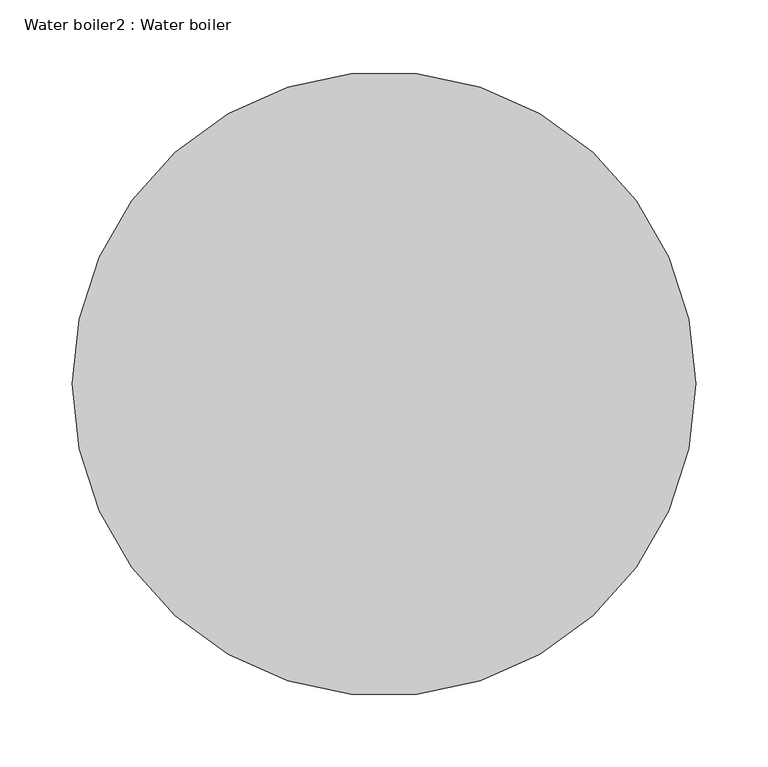
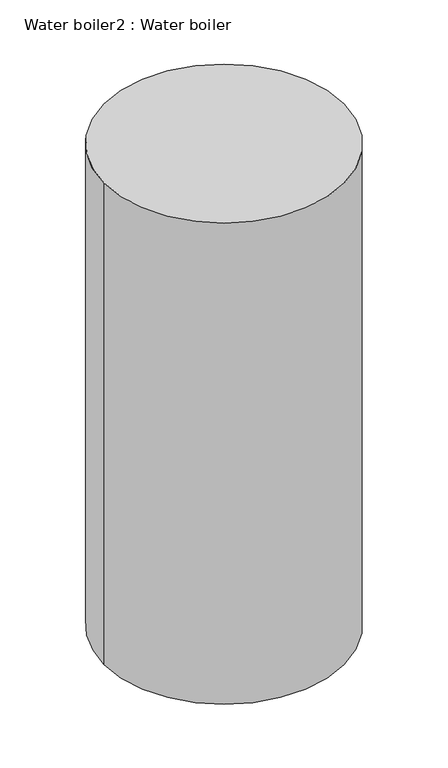
"""IFC4 building model written with IfcOpenShell, lengths in millimetres: proxy geometry, Water boiler2 : Water boiler."""

from ifc_helpers import new_model, si_unit, point, frame, frame_2d, origin, place, context, project, spatial, circle_curve, trimmed, segment, composite_curve, outline, extrude, source, transform, mapped, element, save


def water_boiler2_water_boiler_54bea4d4(model_context):
    return source(origin(), model_context, "Body", "SweptSolid", [
        extrude(outline(composite_curve([segment(trimmed(circle_curve(frame_2d((25724.6370052, 10998.0325125)), 215.9), [point((25508.7370052, 10998.0325125))], [point((25940.5370052, 10998.0325125))], False, "CARTESIAN"), True, "CONTINUOUS"), segment(trimmed(circle_curve(frame_2d((25724.6370052, 10998.0325125)), 215.9), [point((25940.5370052, 10998.0325125))], [point((25508.7370052, 10998.0325125))], False, "CARTESIAN"), True, "CONTINUOUS")], self_intersect=False)), frame((0.0, 0.0, 2832.1), z_axis=(0.0, 0.0, 1.0), x_axis=(1.0, 0.0, 0.0)), (0.0, 0.0, 1.0), 914.4),
    ])


if __name__ == "__main__":
    model = new_model("IFC4")
    model_context = context("Model", 3, world=origin())
    ifc_project = project(units=[si_unit("LENGTHUNIT", "METRE", prefix="MILLI")], contexts=[model_context])
    site = spatial("IfcSite", under=ifc_project)
    building = spatial("IfcBuilding", under=site)
    placement = place(None, origin())
    water_boiler2_water_boiler_shape = water_boiler2_water_boiler_54bea4d4(model_context)
    element("IfcBuildingElementProxy", 1, Name="Water boiler2 : Water boiler", ObjectType="Water boiler2 : Water boiler", at=placement, inside=building, context=model_context, shape_type="MappedRepresentation", body=[
        mapped(water_boiler2_water_boiler_shape, transform((0.0, 0.0, 0.0), x_axis=(1.0, 0.0, 0.0), y_axis=(0.0, 1.0, 0.0), z_axis=(0.0, 0.0, 1.0))),
    ])
    save(model, "model.ifc")
